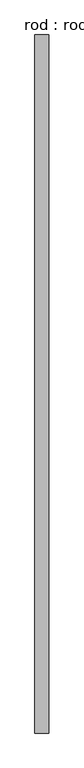
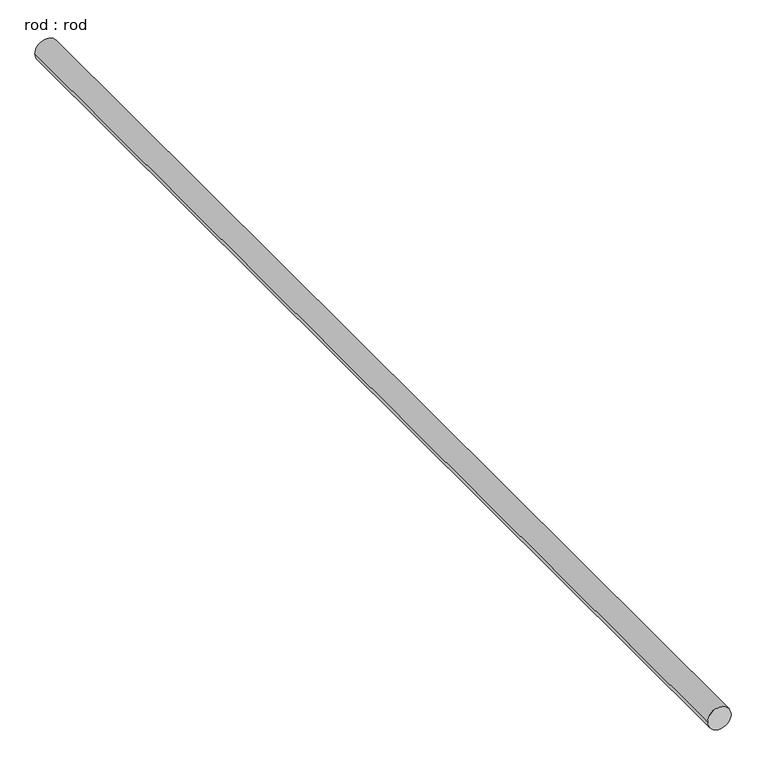
"""IFC4 building model written with IfcOpenShell, lengths in millimetres: proxy geometry, rod : rod."""

import ifcopenshell
import ifcopenshell.guid

model = None  # the IFC model being written
_history = None  # IfcOwnerHistory: only IFC2X3 demands one
_inside = {}  # id of a spatial element -> (the spatial element, [elements in it])
_under = {}  # id of a project, library or spatial element -> (it, [spatial elements below it])
_declared = {}  # id of a project -> (the project, [libraries it declares])
_typed = {}  # id of a type object -> (the type object, [elements of that type])
_made_of = {}  # id of a material, layer set ... -> (it, [elements and type objects made of it])


def new_model(schema):
    """Start an empty IFC model of exactly this schema.

    Asked for "IFC4X3", IfcOpenShell would pick the latest addendum, in which some entities
    have other attributes; the version numbers below select the first issue.
    IFC2X3 requires an IfcOwnerHistory on every rooted entity: one is made here for all.
    """
    global model, _history
    if schema == "IFC4X3":
        model = ifcopenshell.file(schema_version=(4, 3, 0, 0))
    else:
        model = ifcopenshell.file(schema=schema)
    _inside.clear()
    _under.clear()
    _declared.clear()
    _typed.clear()
    _made_of.clear()
    _history = None
    if model.schema == "IFC2X3":
        org = make("IfcOrganization", Name="unknown")
        user = make(
            "IfcPersonAndOrganization",
            ThePerson=make("IfcPerson", FamilyName="unknown"),
            TheOrganization=org,
        )
        app = make(
            "IfcApplication",
            ApplicationDeveloper=org,
            Version="unknown",
            ApplicationFullName="unknown",
            ApplicationIdentifier="unknown",
        )
        _history = make(
            "IfcOwnerHistory",
            OwningUser=user,
            OwningApplication=app,
            ChangeAction="ADDED",
            CreationDate=0,
        )
    return model


def make(cls, **values):
    """One entity of the class cls with the attributes given. An attribute that is None is left unset."""
    return model.create_entity(
        cls, **{name: value for name, value in values.items() if value is not None}
    )


def rooted(cls, **values):
    """An entity with a GlobalId (a new one), such as an element, a storey or a relation."""
    return make(cls, GlobalId=ifcopenshell.guid.new(), OwnerHistory=_history, **values)


def si_unit(unit_type, name, prefix=None):
    """IfcSIUnit, for example si_unit("LENGTHUNIT", "METRE", prefix="MILLI")."""
    return make("IfcSIUnit", UnitType=unit_type, Prefix=prefix, Name=name)


def assignment(units):
    """IfcUnitAssignment: the units of a project."""
    return None if units is None else make("IfcUnitAssignment", Units=units)


def point(xyz):
    """IfcCartesianPoint."""
    return None if xyz is None else make("IfcCartesianPoint", Coordinates=xyz)


def direction(xyz):
    """IfcDirection."""
    return None if xyz is None else make("IfcDirection", DirectionRatios=xyz)


def frame(location, z_axis=None, x_axis=None):
    """IfcAxis2Placement3D, a coordinate frame: its origin and axes. An axis left out is left unset."""
    return make(
        "IfcAxis2Placement3D",
        Location=point(location),
        Axis=direction(z_axis),
        RefDirection=direction(x_axis),
    )


def frame_2d(location, x_axis=None):
    """IfcAxis2Placement2D, a coordinate frame in the plane: its origin and x axis."""
    return make(
        "IfcAxis2Placement2D", Location=point(location), RefDirection=direction(x_axis)
    )


def origin():
    """The frame at (0, 0, 0) with its axes left unset."""
    return frame((0.0, 0.0, 0.0))


def place(relative_to, where):
    """IfcLocalPlacement: puts the frame where relative to a parent placement (None: the world)."""
    return make(
        "IfcLocalPlacement", PlacementRelTo=relative_to, RelativePlacement=where
    )


def context(
    kind, dimensions, precision=None, world=None, true_north=None, identifier=None
):
    """IfcGeometricRepresentationContext, for example the 3D "Model" context."""
    return make(
        "IfcGeometricRepresentationContext",
        ContextIdentifier=identifier,
        ContextType=kind,
        CoordinateSpaceDimension=dimensions,
        Precision=precision,
        WorldCoordinateSystem=world,
        TrueNorth=true_north,
    )


def project(units=None, contexts=None):
    """IfcProject with its units and contexts."""
    return rooted(
        "IfcProject",
        Name="project",
        RepresentationContexts=contexts,
        UnitsInContext=assignment(units),
    )


def spatial(cls, under=None, at=None, **own):
    """A site, building, storey or space (cls), placed at a placement, below another one or the project."""
    s = rooted(cls, ObjectPlacement=at, **own)
    if under is not None:
        _under.setdefault(under.id(), (under, []))[1].append(s)
    return s


def circle_curve(where, radius):
    """IfcCircle in the frame where."""
    return make("IfcCircle", Position=where, Radius=radius)


def trimmed(basis, trim1, trim2, sense, master):
    """IfcTrimmedCurve: the piece of a basis curve between two trims."""
    return make(
        "IfcTrimmedCurve",
        BasisCurve=basis,
        Trim1=trim1,
        Trim2=trim2,
        SenseAgreement=sense,
        MasterRepresentation=master,
    )


def segment(curve, same_sense, transition):
    """IfcCompositeCurveSegment."""
    return make(
        "IfcCompositeCurveSegment",
        Transition=transition,
        SameSense=same_sense,
        ParentCurve=curve,
    )


def composite_curve(segments, self_intersect=None):
    """IfcCompositeCurve: segments joined end to end."""
    return make("IfcCompositeCurve", Segments=segments, SelfIntersect=self_intersect)


def outline(outer, holes=None, kind="AREA"):
    """IfcArbitraryClosedProfileDef: a profile drawn as a closed curve; with holes, ...WithVoids."""
    if holes is None:
        return make("IfcArbitraryClosedProfileDef", ProfileType=kind, OuterCurve=outer)
    return make(
        "IfcArbitraryProfileDefWithVoids",
        ProfileType=kind,
        OuterCurve=outer,
        InnerCurves=holes,
    )


def extrude(swept, where, along, depth):
    """IfcExtrudedAreaSolid: the profile swept, set in the frame where, extruded along a direction by depth."""
    return make(
        "IfcExtrudedAreaSolid",
        SweptArea=swept,
        Position=where,
        ExtrudedDirection=direction(along),
        Depth=depth,
    )


def shape(context_of_items, identifier, shape_type, items):
    """IfcShapeRepresentation: the items that make up one representation, for example the "Body"."""
    return make(
        "IfcShapeRepresentation",
        ContextOfItems=context_of_items,
        RepresentationIdentifier=identifier,
        RepresentationType=shape_type,
        Items=items,
    )


def source(mapping_origin, context_of_items, identifier, shape_type, items):
    """IfcRepresentationMap: a shape defined once, which mapped items show again and again."""
    return make(
        "IfcRepresentationMap",
        MappingOrigin=mapping_origin,
        MappedRepresentation=shape(context_of_items, identifier, shape_type, items),
    )


def transform(
    local_origin,
    x_axis=None,
    y_axis=None,
    z_axis=None,
    scale=None,
    scale2=None,
    scale3=None,
    uniform=True,
):
    """IfcCartesianTransformationOperator3D, or its non-uniform kind. x_axis, y_axis, z_axis: its Axis1, 2, 3."""
    if uniform:
        return make(
            "IfcCartesianTransformationOperator3D",
            Axis1=direction(x_axis),
            Axis2=direction(y_axis),
            LocalOrigin=point(local_origin),
            Scale=scale,
            Axis3=direction(z_axis),
        )
    return make(
        "IfcCartesianTransformationOperator3DnonUniform",
        Axis1=direction(x_axis),
        Axis2=direction(y_axis),
        LocalOrigin=point(local_origin),
        Scale=scale,
        Axis3=direction(z_axis),
        Scale2=scale2,
        Scale3=scale3,
    )


def mapped(mapping_source, mapping_target):
    """IfcMappedItem: shows the shape of a source again, moved by a transform."""
    return make(
        "IfcMappedItem", MappingSource=mapping_source, MappingTarget=mapping_target
    )


def made_of(thing, what):
    """Note that an element or type object is made of a material, layer set ...; save() writes the relation."""
    if what is not None:
        _made_of.setdefault(what.id(), (what, []))[1].append(thing)
    return thing


def element(
    cls,
    number,
    at=None,
    inside=None,
    cuts=None,
    type_object=None,
    material=None,
    context=None,
    identifier="Body",
    shape_type=None,
    held_by="IfcProductDefinitionShape",
    body=None,
    shapes=None,
    **own,
):
    """One element of the class cls, such as IfcWall. Its Tag is "e" and its number.

    at: its placement. inside: the storey or other place that contains it. cuts: it is an
    opening in that element (IfcRelVoidsElement). A single representation is given by context,
    identifier, shape_type and body (its items); several are given by shapes. held_by: the class
    of the entity that holds the representations. save() writes the other relations.
    """
    e = rooted(cls, Tag="e%d" % number, ObjectPlacement=at, **own)
    if body is not None:
        shapes = [shape(context, identifier, shape_type, body)]
    if shapes is not None:
        e.Representation = make(held_by, Representations=shapes)
    if inside is not None:
        _inside.setdefault(inside.id(), (inside, []))[1].append(e)
    if cuts is not None:
        rooted(
            "IfcRelVoidsElement", RelatingBuildingElement=cuts, RelatedOpeningElement=e
        )
    if type_object is not None:
        _typed.setdefault(type_object.id(), (type_object, []))[1].append(e)
    return made_of(e, material)


def aggregate(whole, parts):
    """IfcRelAggregates: a whole, such as a stair, and the parts it consists of."""
    return rooted("IfcRelAggregates", RelatingObject=whole, RelatedObjects=parts)


def save(model, path):
    """Write the relations noted so far, then the file.

    IfcRelAggregates (storeys below a building ...), IfcRelContainedInSpatialStructure (elements
    in a storey), IfcRelDefinesByType, IfcRelAssociatesMaterial and IfcRelDeclares: one each for
    every whole, place, type object, material and project.
    """
    for whole, parts in _under.values():
        aggregate(whole, parts)
    for where, things in _inside.values():
        rooted(
            "IfcRelContainedInSpatialStructure",
            RelatedElements=things,
            RelatingStructure=where,
        )
    for kind, things in _typed.values():
        rooted("IfcRelDefinesByType", RelatedObjects=things, RelatingType=kind)
    for what, things in _made_of.values():
        rooted("IfcRelAssociatesMaterial", RelatedObjects=things, RelatingMaterial=what)
    for by, libraries in _declared.values():
        rooted("IfcRelDeclares", RelatingContext=by, RelatedDefinitions=libraries)
    model.write(path)


def rod_rod_f9bd0e5a(model_context):
    return source(origin(), model_context, "Body", "SweptSolid", [
        extrude(outline(composite_curve([segment(trimmed(circle_curve(frame_2d((0.0108462, 0.0)), 200.0), [point((0.0108462, 200.0))], [point((0.0108462, -200.0))], False, "CARTESIAN"), True, "CONTINUOUS"), segment(trimmed(circle_curve(frame_2d((0.0108462, 0.0)), 200.0), [point((0.0108462, -200.0))], [point((0.0108462, 200.0))], False, "CARTESIAN"), True, "CONTINUOUS")], self_intersect=False)), frame((0.0, -5857.2713847, 0.0), z_axis=(0.0, 1.0, 0.0), x_axis=(0.0, 0.0, 1.0)), (0.0, 0.0, 1.0), 19900.0),
    ])


if __name__ == "__main__":
    model = new_model("IFC4")
    model_context = context("Model", 3, world=origin())
    ifc_project = project(units=[si_unit("LENGTHUNIT", "METRE", prefix="MILLI")], contexts=[model_context])
    site = spatial("IfcSite", under=ifc_project)
    building = spatial("IfcBuilding", under=site)
    placement = place(None, origin())
    rod_rod_shape = rod_rod_f9bd0e5a(model_context)
    element("IfcBuildingElementProxy", 1, Name="rod : rod", ObjectType="rod : rod", at=placement, inside=building, context=model_context, shape_type="MappedRepresentation", body=[
        mapped(rod_rod_shape, transform((0.0, 0.0, 0.0), x_axis=(1.0, 0.0, 0.0), y_axis=(0.0, 1.0, 0.0), z_axis=(0.0, 0.0, 1.0))),
    ])
    save(model, "model.ifc")

# Revit data of these elements
# Type "rod : rod"
#   Default Elevation = 0
